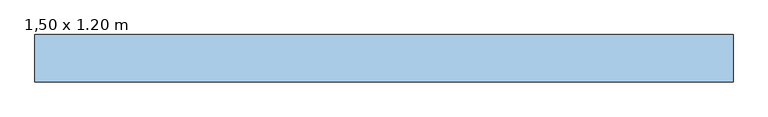
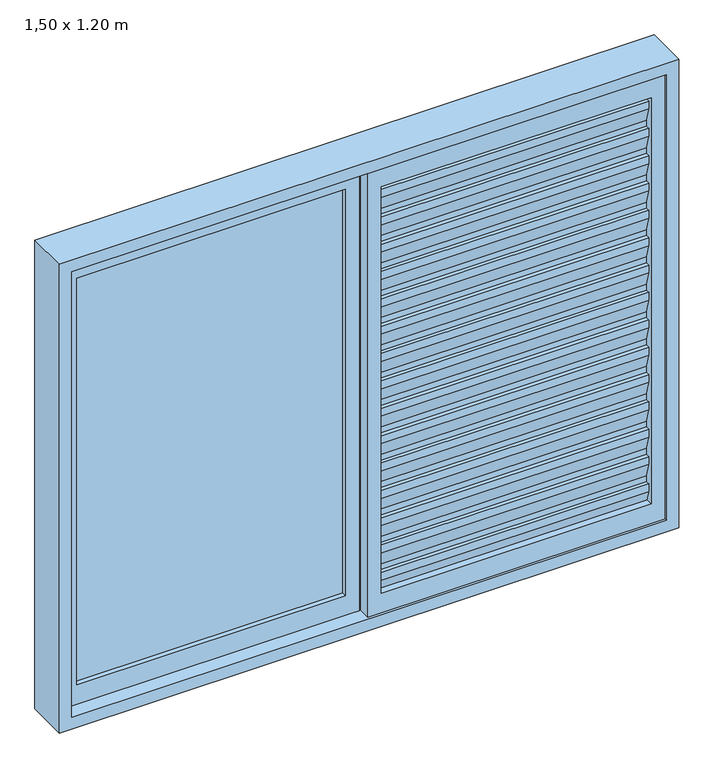
"""IFC4 building model written with IfcOpenShell, lengths in millimetres: window geometry, Janela veneziana de correr - 3 Folhas : 1,50 x 1.20 m."""

from ifc_helpers import new_model, si_unit, frame, origin, place, context, project, spatial, polyline, outline, extrude, source, transform, mapped, element, save


def window_1_50_x_1_20_m_9607e01b(model_context):
    return source(origin(), model_context, "Body", "SweptSolid", [
        extrude(outline(polyline([(-35.3328675, 1024.8599451), (-25.3328675, 1024.8599451), (-25.3328675, 1039.8599451), (-35.3328675, 1074.8599451), (-35.3328675, 1094.8599451), (-25.3328675, 1094.8599451), (-25.3328675, 1109.8599451), (-35.3328675, 1144.8599451), (-35.3328675, 1164.8599451), (-25.3328675, 1164.8599451), (-25.3328675, 1179.8599451), (-35.3328675, 1214.8599451), (-35.3328675, 1234.8599451), (-25.3328675, 1234.8599451), (-25.3328675, 1249.8599451), (-35.3328675, 1284.8599451), (-35.3328675, 1304.8599451), (-25.3328675, 1304.8599451), (-25.3328675, 1319.8599451), (-35.3328675, 1354.8599451), (-35.3328675, 1374.8599451), (-25.3328675, 1374.8599451), (-25.3328675, 1389.8599451), (-35.3328675, 1424.8599451), (-35.3328675, 1444.8599451), (-25.3328675, 1444.8599451), (-25.3328675, 1459.8599451), (-35.3328675, 1494.8599451), (-35.3328675, 1514.8599451), (-25.3328675, 1514.8599451), (-25.3328675, 1529.8599451), (-35.3328675, 1564.8599451), (-35.3328675, 1584.8599451), (-25.3328675, 1584.8599451), (-25.3328675, 1599.8599451), (-35.3328675, 1634.8599451), (-35.3328675, 1654.8599451), (-25.3328675, 1654.8599451), (-25.3328675, 1669.8599451), (-35.3328675, 1704.8599451), (-35.3328675, 1724.8599451), (-25.3328675, 1724.8599451), (-25.3328675, 1739.8599451), (-35.3328675, 1774.8599451), (-35.3328675, 1794.8599451), (-25.3328675, 1794.8599451), (-25.3328675, 1809.8599451), (-35.3328675, 1844.8599451), (-35.3328675, 1864.8599451), (-25.3328675, 1864.8599451), (-25.3328675, 1879.8599451), (-35.3328675, 1914.8599451), (-35.3328675, 1934.8599451), (-25.3328675, 1934.8599451), (-25.3328675, 1949.8599451), (-35.3328675, 1984.8599451), (-35.3328675, 2004.8599451), (-25.3328675, 2004.8599451), (-25.3328675, 2019.8599451), (-24.3328675, 2020.0), (-24.3328675, 2003.8599451), (-34.3328675, 2003.8599451), (-34.3328675, 1985.0), (-24.3328675, 1950.0), (-24.3328675, 1933.8599451), (-34.3328675, 1933.8599451), (-34.3328675, 1915.0), (-24.3328675, 1880.0), (-24.3328675, 1863.8599451), (-34.3328675, 1863.8599451), (-34.3328675, 1845.0), (-24.3328675, 1810.0), (-24.3328675, 1793.8599451), (-34.3328675, 1793.8599451), (-34.3328675, 1775.0), (-24.3328675, 1740.0), (-24.3328675, 1723.8599451), (-34.3328675, 1723.8599451), (-34.3328675, 1705.0), (-24.3328675, 1670.0), (-24.3328675, 1653.8599451), (-34.3328675, 1653.8599451), (-34.3328675, 1635.0), (-24.3328675, 1600.0), (-24.3328675, 1583.8599451), (-34.3328675, 1583.8599451), (-34.3328675, 1565.0), (-24.3328675, 1530.0), (-24.3328675, 1513.8599451), (-34.3328675, 1513.8599451), (-34.3328675, 1495.0), (-24.3328675, 1460.0), (-24.3328675, 1443.8599451), (-34.3328675, 1443.8599451), (-34.3328675, 1425.0), (-24.3328675, 1390.0), (-24.3328675, 1373.8599451), (-34.3328675, 1373.8599451), (-34.3328675, 1355.0), (-24.3328675, 1320.0), (-24.3328675, 1303.8599451), (-34.3328675, 1303.8599451), (-34.3328675, 1285.0), (-24.3328675, 1250.0), (-24.3328675, 1233.8599451), (-34.3328675, 1233.8599451), (-34.3328675, 1215.0), (-24.3328675, 1180.0), (-24.3328675, 1163.8599451), (-34.3328675, 1163.8599451), (-34.3328675, 1145.0), (-24.3328675, 1110.0), (-24.3328675, 1093.8599451), (-34.3328675, 1093.8599451), (-34.3328675, 1075.0), (-24.3328675, 1040.0), (-24.3328675, 1023.8599451), (-34.3328675, 1023.8599451), (-34.3328675, 1005.0), (-27.1900104, 980.0), (-28.2300261, 980.0), (-35.3328675, 1004.8599451), (-35.3328675, 1024.8599451)])), frame((33.4363773, 0.0, 0.0), z_axis=(1.0, 0.0, 0.0), x_axis=(0.0, 1.0, 0.0)), (0.0, 0.0, 1.0), 653.1),
        extrude(outline(polyline([(2070.0, 0.0), (930.0, 0.0), (930.0, 720.0), (2070.0, 720.0), (2070.0, 0.0)]), holes=[polyline([(2020.0, 33.4636227), (2020.0, 686.5363773), (980.0, 686.5363773), (980.0, 33.4636227), (2020.0, 33.4636227)])]), frame((0.0, -46.0, 0.0), z_axis=(0.0, 1.0, 0.0), x_axis=(0.0, 0.0, 1.0)), (0.0, 0.0, 1.0), 30.0),
        extrude(outline(polyline([(27.9809279, 1024.8599451), (37.9809279, 1024.8599451), (37.9809279, 1039.8599451), (27.9809279, 1074.8599451), (27.9809279, 1094.8599451), (37.9809279, 1094.8599451), (37.9809279, 1109.8599451), (27.9809279, 1144.8599451), (27.9809279, 1164.8599451), (37.9809279, 1164.8599451), (37.9809279, 1179.8599451), (27.9809279, 1214.8599451), (27.9809279, 1234.8599451), (37.9809279, 1234.8599451), (37.9809279, 1249.8599451), (27.9809279, 1284.8599451), (27.9809279, 1304.8599451), (37.9809279, 1304.8599451), (37.9809279, 1319.8599451), (27.9809279, 1354.8599451), (27.9809279, 1374.8599451), (37.9809279, 1374.8599451), (37.9809279, 1389.8599451), (27.9809279, 1424.8599451), (27.9809279, 1444.8599451), (37.9809279, 1444.8599451), (37.9809279, 1459.8599451), (27.9809279, 1494.8599451), (27.9809279, 1514.8599451), (37.9809279, 1514.8599451), (37.9809279, 1529.8599451), (27.9809279, 1564.8599451), (27.9809279, 1584.8599451), (37.9809279, 1584.8599451), (37.9809279, 1599.8599451), (27.9809279, 1634.8599451), (27.9809279, 1654.8599451), (37.9809279, 1654.8599451), (37.9809279, 1669.8599451), (27.9809279, 1704.8599451), (27.9809279, 1724.8599451), (37.9809279, 1724.8599451), (37.9809279, 1739.8599451), (27.9809279, 1774.8599451), (27.9809279, 1794.8599451), (37.9809279, 1794.8599451), (37.9809279, 1809.8599451), (27.9809279, 1844.8599451), (27.9809279, 1864.8599451), (37.9809279, 1864.8599451), (37.9809279, 1879.8599451), (27.9809279, 1914.8599451), (27.9809279, 1934.8599451), (37.9809279, 1934.8599451), (37.9809279, 1949.8599451), (27.9809279, 1984.8599451), (27.9809279, 2004.8599451), (37.9809279, 2004.8599451), (37.9809279, 2019.8599451), (38.9809279, 2020.0), (38.9809279, 2003.8599451), (28.9809279, 2003.8599451), (28.9809279, 1985.0), (38.9809279, 1950.0), (38.9809279, 1933.8599451), (28.9809279, 1933.8599451), (28.9809279, 1915.0), (38.9809279, 1880.0), (38.9809279, 1863.8599451), (28.9809279, 1863.8599451), (28.9809279, 1845.0), (38.9809279, 1810.0), (38.9809279, 1793.8599451), (28.9809279, 1793.8599451), (28.9809279, 1775.0), (38.9809279, 1740.0), (38.9809279, 1723.8599451), (28.9809279, 1723.8599451), (28.9809279, 1705.0), (38.9809279, 1670.0), (38.9809279, 1653.8599451), (28.9809279, 1653.8599451), (28.9809279, 1635.0), (38.9809279, 1600.0), (38.9809279, 1583.8599451), (28.9809279, 1583.8599451), (28.9809279, 1565.0), (38.9809279, 1530.0), (38.9809279, 1513.8599451), (28.9809279, 1513.8599451), (28.9809279, 1495.0), (38.9809279, 1460.0), (38.9809279, 1443.8599451), (28.9809279, 1443.8599451), (28.9809279, 1425.0), (38.9809279, 1390.0), (38.9809279, 1373.8599451), (28.9809279, 1373.8599451), (28.9809279, 1355.0), (38.9809279, 1320.0), (38.9809279, 1303.8599451), (28.9809279, 1303.8599451), (28.9809279, 1285.0), (38.9809279, 1250.0), (38.9809279, 1233.8599451), (28.9809279, 1233.8599451), (28.9809279, 1215.0), (38.9809279, 1180.0), (38.9809279, 1163.8599451), (28.9809279, 1163.8599451), (28.9809279, 1145.0), (38.9809279, 1110.0), (38.9809279, 1093.8599451), (28.9809279, 1093.8599451), (28.9809279, 1075.0), (38.9809279, 1040.0), (38.9809279, 1023.8599451), (28.9809279, 1023.8599451), (28.9809279, 1005.0), (36.123785, 980.0), (35.0837693, 980.0), (27.9809279, 1004.8599451), (27.9809279, 1024.8599451)])), frame((33.4363773, 0.0, 0.0), z_axis=(1.0, 0.0, 0.0), x_axis=(0.0, 1.0, 0.0)), (0.0, 0.0, 1.0), 653.1),
        extrude(outline(polyline([(2070.0, 0.0), (930.0, 0.0), (930.0, 720.0), (2070.0, 720.0), (2070.0, 0.0)]), holes=[polyline([(2020.0, 33.4636227), (2020.0, 686.5363773), (980.0, 686.5363773), (980.0, 33.4636227), (2020.0, 33.4636227)])]), frame((0.0, 17.3137954, 0.0), z_axis=(0.0, 1.0, 0.0), x_axis=(0.0, 0.0, 1.0)), (0.0, 0.0, 1.0), 30.0),
        extrude(outline(polyline([(-686.5363773, 2.8137954), (-36.5363773, 2.8137954), (-36.5363773, -4.1862046), (-686.5363773, -4.1862046), (-686.5363773, 2.8137954)])), frame((0.0, 0.0, 980.0), z_axis=(0.0, 0.0, 1.0), x_axis=(1.0, 0.0, 0.0)), (0.0, 0.0, 1.0), 1040.0),
        extrude(outline(polyline([(2070.0, -3.0727546), (2070.0, -720.0), (930.0, -720.0), (930.0, -3.0727546), (2070.0, -3.0727546)]), holes=[polyline([(2020.0, -36.5363773), (980.0, -36.5363773), (980.0, -686.5363773), (2020.0, -686.5363773), (2020.0, -36.5363773)])]), frame((0.0, -15.6862046, 0.0), z_axis=(0.0, 1.0, 0.0), x_axis=(0.0, 0.0, 1.0)), (0.0, 0.0, 1.0), 30.0),
        extrude(outline(polyline([(2100.0, 750.0), (2100.0, -750.0), (900.0, -750.0), (900.0, 750.0), (2100.0, 750.0)]), holes=[polyline([(2070.0, 720.0), (930.0, 720.0), (930.0, -720.0), (2070.0, -720.0), (2070.0, 720.0)])]), frame((0.0, -51.6862046, 0.0), z_axis=(0.0, 1.0, 0.0), x_axis=(0.0, 0.0, 1.0)), (0.0, 0.0, 1.0), 102.0),
    ])


if __name__ == "__main__":
    model = new_model("IFC4")
    model_context = context("Model", 3, world=origin())
    ifc_project = project(units=[si_unit("LENGTHUNIT", "METRE", prefix="MILLI")], contexts=[model_context])
    site = spatial("IfcSite", under=ifc_project)
    building = spatial("IfcBuilding", under=site)
    placement = place(None, origin())
    window_1_50_x_1_20_m_shape = window_1_50_x_1_20_m_9607e01b(model_context)
    element("IfcWindow", 1, ObjectType="Janela veneziana de correr - 3 Folhas : 1,50 x 1.20 m", at=placement, inside=building, context=model_context, shape_type="MappedRepresentation", body=[
        mapped(window_1_50_x_1_20_m_shape, transform((0.0, 0.0, 0.0), x_axis=(1.0, 0.0, 0.0), y_axis=(0.0, 1.0, 0.0), z_axis=(0.0, 0.0, 1.0))),
    ])
    save(model, "model.ifc")

# Revit data of these elements
# Type "Janela veneziana de correr - 3 Folhas : 1,50 x 1.20 m"
#   Type Mark = "J23"
#   Analytic Construction = "<Nenhum>"
#   Largura Vão = 0.685 m
#   Largura Veneziana = 0.6531 m
#   L_est_v marco = 0.033464 m
#   L_est_h_marco = 0.050 m
#   L_contramarco = 0.030 m
#   Height = 1.200 m
#   Altura-padrão do peitoril = 0.900 m
#   Width = 1.500 m
#   Material estrutura = Metal - Alumínio
#   Material Veneziana = Metal - Alumínio
#   Material Quadro = Metal - Alumínio
#   Material Painel = Vidro
#   Wall Closure = (empty or 0)
# Element 1 (IfcWindow, "Janela veneziana de correr - 3 Folhas : 1,50 x 1.20 m")
#   Materials on its faces: "Metal - Alumínio", "Vidro"
# Materials
#   "Metal - Alumínio": class "Metal", colour RGB 247 247 247, transparency 0
#   "Vidro": class "Vidro", colour RGB 0 128 192, transparency 0.9
